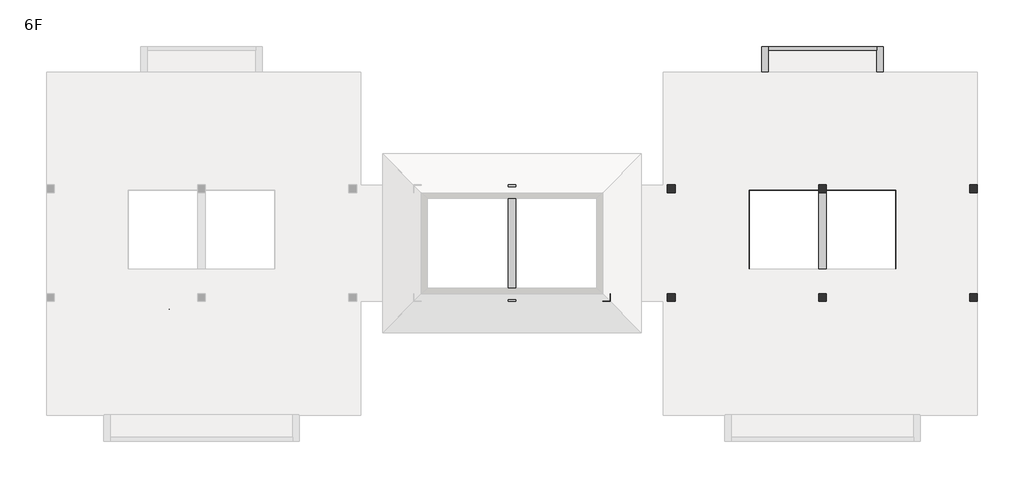
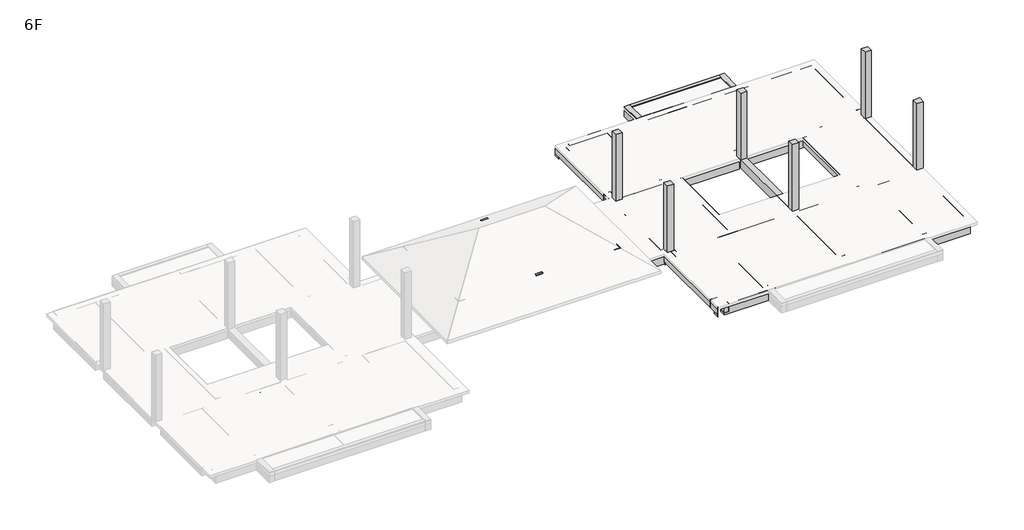
# One storey, part 2 of 2: 33 beams, 10 columns, 1 proxy.
# Revit data of these elements (continued)
# Element 13 (IfcBeam, "M_Concrete-Rectangular Beam : 250x500")
#   Comments = ""
#   COF_GEN__Name = "DP2A"
#   Structural Material = Concrete, Cast-in-Place gray
#   Phase Created = New Construction
#   Materials on its faces: "Concrete, Cast-in-Place gray"
# Element 14 (IfcBeam, "M_Concrete-Rectangular Beam : 300x400")
#   Comments = ""
#   COF_CON__WorkItemNumber = "SH3-A-03F"
#   COF_GEN__Name = "DT1"
#   Structural Material = Concrete, Cast-in-Place gray
#   Phase Created = New Construction
#   Materials on its faces: "Concrete, Cast-in-Place gray"
# Elements 15, 16, 17 (IfcBeam, "M_Concrete-Rectangular Beam : 300x400")
#   Comments = ""
#   COF_CON__WorkItemNumber = "SH3-A-03F"
#   COF_GEN__Name = "D7"
#   Structural Material = Concrete, Cast-in-Place gray
#   Phase Created = New Construction
#   Materials on its faces: "Concrete, Cast-in-Place gray"
# Elements 18, 19, 20 (IfcBeam, "M_Concrete-Rectangular Beam : 300x400")
#   Comments = ""
#   COF_CON__WorkItemNumber = "SH3-A-03F"
#   COF_GEN__Name = "D3"
#   Structural Material = Concrete, Cast-in-Place gray
#   Phase Created = New Construction
#   Materials on its faces: "Concrete, Cast-in-Place gray"
# Elements 21, 22 (IfcBeam, "M_Concrete-Rectangular Beam : 300x500")
#   Comments = ""
#   COF_CON__WorkItemNumber = "SH3-A-03F"
#   COF_GEN__Name = "D2B"
#   Structural Material = Concrete, Cast-in-Place gray
#   Phase Created = New Construction
#   Materials on its faces: "Concrete, Cast-in-Place gray"
# Elements 23, 24, 25, 26, 27, 28, 29, 30 (IfcBeam, "M_Concrete-Rectangular Beam : 300x500")
#   Comments = ""
#   COF_CON__WorkItemNumber = "SH3-A-03F"
#   COF_GEN__Name = "D2"
#   Structural Material = Concrete, Cast-in-Place gray
#   Phase Created = New Construction
#   Materials on its faces: "Concrete, Cast-in-Place gray"
# Elements 31, 32, 33 (IfcBeam, "M_Concrete-Rectangular Beam : 500x400")
#   Comments = ""
#   COF_CON__WorkItemNumber = "SH3-A-03F"
#   COF_GEN__Name = "D3A"
#   Structural Material = Concrete, Cast-in-Place gray
#   Phase Created = New Construction
#   Materials on its faces: "Concrete, Cast-in-Place gray"
# Element 34 (IfcBuildingElementProxy, "M_Support - Metal - Circular : M_Support - Metal - Circular")
#   built-in parameter 1152165 = 0.246063 (stored number, unit not read)
#   Materials on its faces: "Aluminum"
# Elements 35, 36 (IfcColumn, "M_Concrete-Rectangular-Column : 300x300")
#   Comments = ""
#   COF_CON__WorkItemNumber = "SH3-A-RF"
#   COF_GEN__Name = "TR1"
#   Structural Material = Concrete, Cast-in-Place gray
#   Phase Created = New Construction
#   Materials on its faces: "Concrete, Cast-in-Place gray"
# Elements 37, 38 (IfcColumn, "M_Concrete-Rectangular-Column : 300x300")
#   Comments = ""
#   COF_CON__WorkItemNumber = "SH3-A-RF"
#   COF_GEN__Name = "TR2"
#   Structural Material = Concrete, Cast-in-Place gray
#   Phase Created = New Construction
#   Materials on its faces: "Concrete, Cast-in-Place gray"
# Elements 39, 40, 43, 44 (IfcColumn, "M_Concrete-Rectangular-Column : 300x300")
#   Comments = ""
#   COF_CON__WorkItemNumber = "SH3-A-RF"
#   COF_GEN__Name = "TR3"
#   Structural Material = Concrete, Cast-in-Place gray
#   Phase Created = New Construction
#   Materials on its faces: "Concrete, Cast-in-Place gray"
# Elements 41, 42 (IfcColumn, "M_Concrete-Rectangular-Column : 300x300")
#   Comments = ""
#   COF_CON__WorkItemNumber = "SH3-A-RF"
#   COF_GEN__Name = "TR4"
#   Structural Material = Concrete, Cast-in-Place gray
#   Phase Created = New Construction
#   Materials on its faces: "Concrete, Cast-in-Place gray"
# Materials
#   "Concrete, Cast-in-Place gray": class "Concrete", colour RGB 207 208 204, transparency 0, Description = "Cast-in-place concrete", Cost = 0
#   "Aluminum": class "Metal", colour RGB 247 247 247, transparency 0, Description = "Aluminum 6061", Cost = 0
